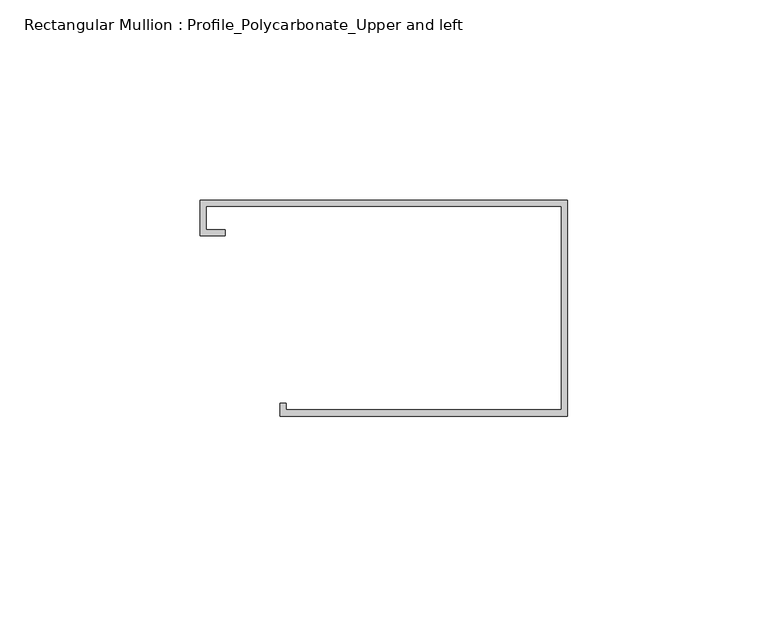
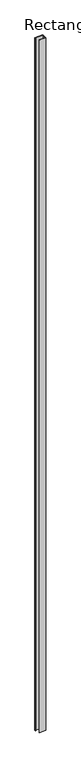
"""IFC4 building model written with IfcOpenShell, lengths in millimetres: member geometry, Rectangular Mullion : Profile_Polycarbonate_Upper and left."""

import ifcopenshell
import ifcopenshell.guid

model = None  # the IFC model being written
_history = None  # IfcOwnerHistory: only IFC2X3 demands one
_inside = {}  # id of a spatial element -> (the spatial element, [elements in it])
_under = {}  # id of a project, library or spatial element -> (it, [spatial elements below it])
_declared = {}  # id of a project -> (the project, [libraries it declares])
_typed = {}  # id of a type object -> (the type object, [elements of that type])
_made_of = {}  # id of a material, layer set ... -> (it, [elements and type objects made of it])


def new_model(schema):
    """Start an empty IFC model of exactly this schema.

    Asked for "IFC4X3", IfcOpenShell would pick the latest addendum, in which some entities
    have other attributes; the version numbers below select the first issue.
    IFC2X3 requires an IfcOwnerHistory on every rooted entity: one is made here for all.
    """
    global model, _history
    if schema == "IFC4X3":
        model = ifcopenshell.file(schema_version=(4, 3, 0, 0))
    else:
        model = ifcopenshell.file(schema=schema)
    _inside.clear()
    _under.clear()
    _declared.clear()
    _typed.clear()
    _made_of.clear()
    _history = None
    if model.schema == "IFC2X3":
        org = make("IfcOrganization", Name="unknown")
        user = make(
            "IfcPersonAndOrganization",
            ThePerson=make("IfcPerson", FamilyName="unknown"),
            TheOrganization=org,
        )
        app = make(
            "IfcApplication",
            ApplicationDeveloper=org,
            Version="unknown",
            ApplicationFullName="unknown",
            ApplicationIdentifier="unknown",
        )
        _history = make(
            "IfcOwnerHistory",
            OwningUser=user,
            OwningApplication=app,
            ChangeAction="ADDED",
            CreationDate=0,
        )
    return model


def make(cls, **values):
    """One entity of the class cls with the attributes given. An attribute that is None is left unset."""
    return model.create_entity(
        cls, **{name: value for name, value in values.items() if value is not None}
    )


def rooted(cls, **values):
    """An entity with a GlobalId (a new one), such as an element, a storey or a relation."""
    return make(cls, GlobalId=ifcopenshell.guid.new(), OwnerHistory=_history, **values)


def si_unit(unit_type, name, prefix=None):
    """IfcSIUnit, for example si_unit("LENGTHUNIT", "METRE", prefix="MILLI")."""
    return make("IfcSIUnit", UnitType=unit_type, Prefix=prefix, Name=name)


def assignment(units):
    """IfcUnitAssignment: the units of a project."""
    return None if units is None else make("IfcUnitAssignment", Units=units)


def point(xyz):
    """IfcCartesianPoint."""
    return None if xyz is None else make("IfcCartesianPoint", Coordinates=xyz)


def direction(xyz):
    """IfcDirection."""
    return None if xyz is None else make("IfcDirection", DirectionRatios=xyz)


def frame(location, z_axis=None, x_axis=None):
    """IfcAxis2Placement3D, a coordinate frame: its origin and axes. An axis left out is left unset."""
    return make(
        "IfcAxis2Placement3D",
        Location=point(location),
        Axis=direction(z_axis),
        RefDirection=direction(x_axis),
    )


def origin():
    """The frame at (0, 0, 0) with its axes left unset."""
    return frame((0.0, 0.0, 0.0))


def place(relative_to, where):
    """IfcLocalPlacement: puts the frame where relative to a parent placement (None: the world)."""
    return make(
        "IfcLocalPlacement", PlacementRelTo=relative_to, RelativePlacement=where
    )


def context(
    kind, dimensions, precision=None, world=None, true_north=None, identifier=None
):
    """IfcGeometricRepresentationContext, for example the 3D "Model" context."""
    return make(
        "IfcGeometricRepresentationContext",
        ContextIdentifier=identifier,
        ContextType=kind,
        CoordinateSpaceDimension=dimensions,
        Precision=precision,
        WorldCoordinateSystem=world,
        TrueNorth=true_north,
    )


def project(units=None, contexts=None):
    """IfcProject with its units and contexts."""
    return rooted(
        "IfcProject",
        Name="project",
        RepresentationContexts=contexts,
        UnitsInContext=assignment(units),
    )


def spatial(cls, under=None, at=None, **own):
    """A site, building, storey or space (cls), placed at a placement, below another one or the project."""
    s = rooted(cls, ObjectPlacement=at, **own)
    if under is not None:
        _under.setdefault(under.id(), (under, []))[1].append(s)
    return s


def polyline(points):
    """IfcPolyline through the points."""
    return make("IfcPolyline", Points=[point(p) for p in points])


def outline(outer, holes=None, kind="AREA"):
    """IfcArbitraryClosedProfileDef: a profile drawn as a closed curve; with holes, ...WithVoids."""
    if holes is None:
        return make("IfcArbitraryClosedProfileDef", ProfileType=kind, OuterCurve=outer)
    return make(
        "IfcArbitraryProfileDefWithVoids",
        ProfileType=kind,
        OuterCurve=outer,
        InnerCurves=holes,
    )


def extrude(swept, where, along, depth):
    """IfcExtrudedAreaSolid: the profile swept, set in the frame where, extruded along a direction by depth."""
    return make(
        "IfcExtrudedAreaSolid",
        SweptArea=swept,
        Position=where,
        ExtrudedDirection=direction(along),
        Depth=depth,
    )


def shape(context_of_items, identifier, shape_type, items):
    """IfcShapeRepresentation: the items that make up one representation, for example the "Body"."""
    return make(
        "IfcShapeRepresentation",
        ContextOfItems=context_of_items,
        RepresentationIdentifier=identifier,
        RepresentationType=shape_type,
        Items=items,
    )


def source(mapping_origin, context_of_items, identifier, shape_type, items):
    """IfcRepresentationMap: a shape defined once, which mapped items show again and again."""
    return make(
        "IfcRepresentationMap",
        MappingOrigin=mapping_origin,
        MappedRepresentation=shape(context_of_items, identifier, shape_type, items),
    )


def transform(
    local_origin,
    x_axis=None,
    y_axis=None,
    z_axis=None,
    scale=None,
    scale2=None,
    scale3=None,
    uniform=True,
):
    """IfcCartesianTransformationOperator3D, or its non-uniform kind. x_axis, y_axis, z_axis: its Axis1, 2, 3."""
    if uniform:
        return make(
            "IfcCartesianTransformationOperator3D",
            Axis1=direction(x_axis),
            Axis2=direction(y_axis),
            LocalOrigin=point(local_origin),
            Scale=scale,
            Axis3=direction(z_axis),
        )
    return make(
        "IfcCartesianTransformationOperator3DnonUniform",
        Axis1=direction(x_axis),
        Axis2=direction(y_axis),
        LocalOrigin=point(local_origin),
        Scale=scale,
        Axis3=direction(z_axis),
        Scale2=scale2,
        Scale3=scale3,
    )


def mapped(mapping_source, mapping_target):
    """IfcMappedItem: shows the shape of a source again, moved by a transform."""
    return make(
        "IfcMappedItem", MappingSource=mapping_source, MappingTarget=mapping_target
    )


def made_of(thing, what):
    """Note that an element or type object is made of a material, layer set ...; save() writes the relation."""
    if what is not None:
        _made_of.setdefault(what.id(), (what, []))[1].append(thing)
    return thing


def element(
    cls,
    number,
    at=None,
    inside=None,
    cuts=None,
    type_object=None,
    material=None,
    context=None,
    identifier="Body",
    shape_type=None,
    held_by="IfcProductDefinitionShape",
    body=None,
    shapes=None,
    **own,
):
    """One element of the class cls, such as IfcWall. Its Tag is "e" and its number.

    at: its placement. inside: the storey or other place that contains it. cuts: it is an
    opening in that element (IfcRelVoidsElement). A single representation is given by context,
    identifier, shape_type and body (its items); several are given by shapes. held_by: the class
    of the entity that holds the representations. save() writes the other relations.
    """
    e = rooted(cls, Tag="e%d" % number, ObjectPlacement=at, **own)
    if body is not None:
        shapes = [shape(context, identifier, shape_type, body)]
    if shapes is not None:
        e.Representation = make(held_by, Representations=shapes)
    if inside is not None:
        _inside.setdefault(inside.id(), (inside, []))[1].append(e)
    if cuts is not None:
        rooted(
            "IfcRelVoidsElement", RelatingBuildingElement=cuts, RelatedOpeningElement=e
        )
    if type_object is not None:
        _typed.setdefault(type_object.id(), (type_object, []))[1].append(e)
    return made_of(e, material)


def aggregate(whole, parts):
    """IfcRelAggregates: a whole, such as a stair, and the parts it consists of."""
    return rooted("IfcRelAggregates", RelatingObject=whole, RelatedObjects=parts)


def save(model, path):
    """Write the relations noted so far, then the file.

    IfcRelAggregates (storeys below a building ...), IfcRelContainedInSpatialStructure (elements
    in a storey), IfcRelDefinesByType, IfcRelAssociatesMaterial and IfcRelDeclares: one each for
    every whole, place, type object, material and project.
    """
    for whole, parts in _under.values():
        aggregate(whole, parts)
    for where, things in _inside.values():
        rooted(
            "IfcRelContainedInSpatialStructure",
            RelatedElements=things,
            RelatingStructure=where,
        )
    for kind, things in _typed.values():
        rooted("IfcRelDefinesByType", RelatedObjects=things, RelatingType=kind)
    for what, things in _made_of.values():
        rooted("IfcRelAssociatesMaterial", RelatedObjects=things, RelatingMaterial=what)
    for by, libraries in _declared.values():
        rooted("IfcRelDeclares", RelatingContext=by, RelatedDefinitions=libraries)
    model.write(path)


def rectangular_mullion_profile_polycarbonate_upper_and_left_4e809100(model_context):
    return source(origin(), model_context, "Body", "SweptSolid", [
        extrude(outline(polyline([(0.0, 28.984575), (0.0, -25.015825), (-71.9836, -25.015825), (-71.9836, -21.840825), (-70.3961, -21.840825), (-70.3961, -23.428325), (-1.5875, -23.428325), (-1.5875, 27.397075), (-90.4113, 27.397075), (-90.4113, 21.580475), (-85.6488, 21.580475), (-85.6488, 19.992975), (-91.9988, 19.992975), (-91.9988, 28.984575), (0.0, 28.984575)])), frame((0.0, 0.0, -8354.1024), z_axis=(0.0, 0.0, 1.0), x_axis=(1.0, 0.0, 0.0)), (0.0, 0.0, 1.0), 8354.1024),
    ])


if __name__ == "__main__":
    model = new_model("IFC4")
    model_context = context("Model", 3, world=origin())
    ifc_project = project(units=[si_unit("LENGTHUNIT", "METRE", prefix="MILLI")], contexts=[model_context])
    site = spatial("IfcSite", under=ifc_project)
    building = spatial("IfcBuilding", under=site)
    placement = place(None, origin())
    rectangular_mullion_profile_polycarbonate_upper_and_left_shape = rectangular_mullion_profile_polycarbonate_upper_and_left_4e809100(model_context)
    element("IfcMember", 1, ObjectType="Rectangular Mullion : Profile_Polycarbonate_Upper and left", at=placement, inside=building, context=model_context, shape_type="MappedRepresentation", body=[
        mapped(rectangular_mullion_profile_polycarbonate_upper_and_left_shape, transform((0.0, 0.0, 0.0), x_axis=(1.0, 0.0, 0.0), y_axis=(0.0, 1.0, 0.0), z_axis=(0.0, 0.0, 1.0))),
    ])
    save(model, "model.ifc")

# Revit data of these elements
# Type "Rectangular Mullion : Profile_Polycarbonate_Upper and left"
#   built-in parameter 1007322 = 0.177167 (stored number, unit not read)
#   built-in parameter 1007321 = 0.00520833 (stored number, unit not read)
#   built-in parameter 1007320 = 0 (stored number, unit not read)
